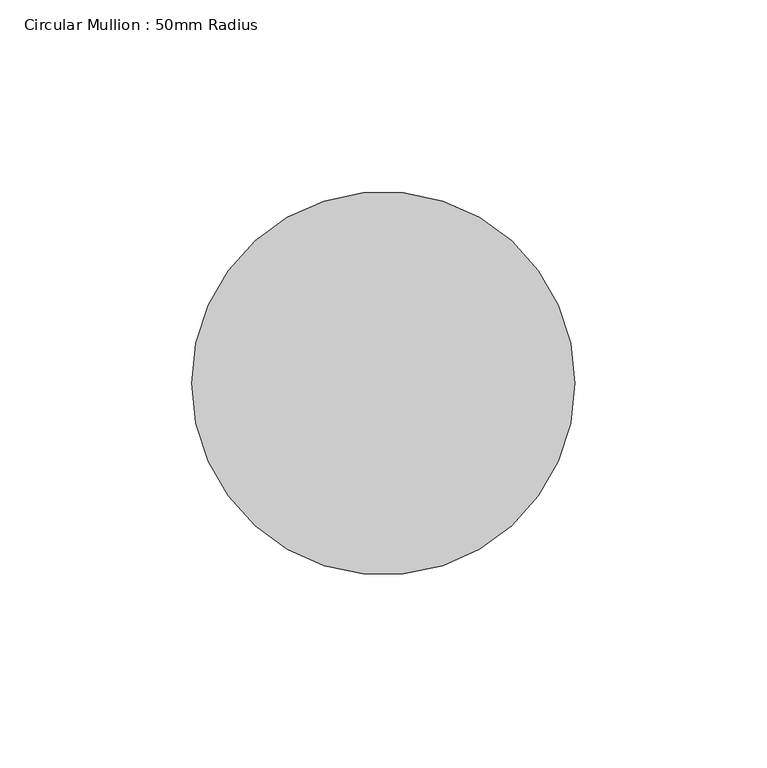
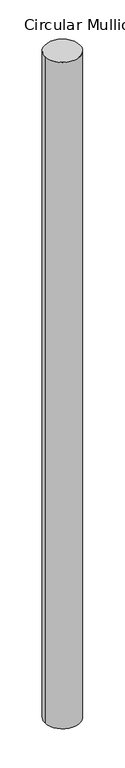
"""IFC4 building model written with IfcOpenShell, lengths in millimetres: member geometry, Circular Mullion : 50mm Radius."""

from ifc_helpers import new_model, si_unit, point, frame, origin, origin_2d, place, context, project, spatial, circle_curve, trimmed, segment, composite_curve, outline, extrude, source, transform, mapped, element, save


def circular_mullion_50mm_radius_5081a5b3(model_context):
    return source(origin(), model_context, "Body", "SweptSolid", [
        extrude(outline(composite_curve([segment(trimmed(circle_curve(origin_2d(), 50.0), [point((50.0, 0.0))], [point((-50.0, 0.0))], False, "CARTESIAN"), True, "CONTINUOUS"), segment(trimmed(circle_curve(origin_2d(), 50.0), [point((-50.0, 0.0))], [point((50.0, 0.0))], False, "CARTESIAN"), True, "CONTINUOUS")], self_intersect=False)), frame((0.0, 0.0, -2000.4049305), z_axis=(0.0, 0.0, 1.0), x_axis=(1.0, 0.0, 0.0)), (0.0, 0.0, 1.0), 2000.4049305),
    ])


if __name__ == "__main__":
    model = new_model("IFC4")
    model_context = context("Model", 3, world=origin())
    ifc_project = project(units=[si_unit("LENGTHUNIT", "METRE", prefix="MILLI")], contexts=[model_context])
    site = spatial("IfcSite", under=ifc_project)
    building = spatial("IfcBuilding", under=site)
    placement = place(None, origin())
    circular_mullion_50mm_radius_shape = circular_mullion_50mm_radius_5081a5b3(model_context)
    element("IfcMember", 1, ObjectType="Circular Mullion : 50mm Radius", at=placement, inside=building, context=model_context, shape_type="MappedRepresentation", body=[
        mapped(circular_mullion_50mm_radius_shape, transform((0.0, 0.0, 0.0), x_axis=(1.0, 0.0, 0.0), y_axis=(0.0, 1.0, 0.0), z_axis=(0.0, 0.0, 1.0))),
    ])
    save(model, "model.ifc")

# Revit data of these elements
# Type "Circular Mullion : 50mm Radius"
#   built-in parameter 1007350 = 0.164042 (stored number, unit not read)
# Element 1 (IfcMember, "Circular Mullion : 50mm Radius")
#   Materials on its faces: "Aluminium"
# Materials
#   "Aluminium": class "Metal", colour RGB 247 247 247, transparency 0, Description = "Aluminium 6061", Cost = 0
